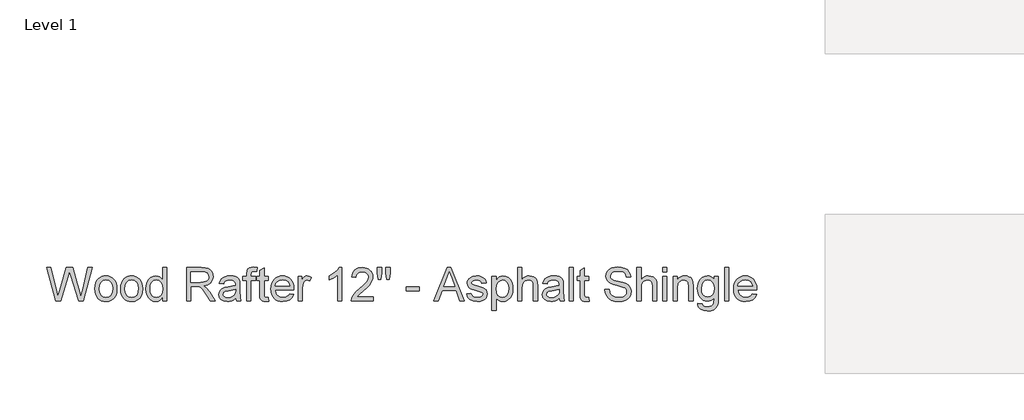
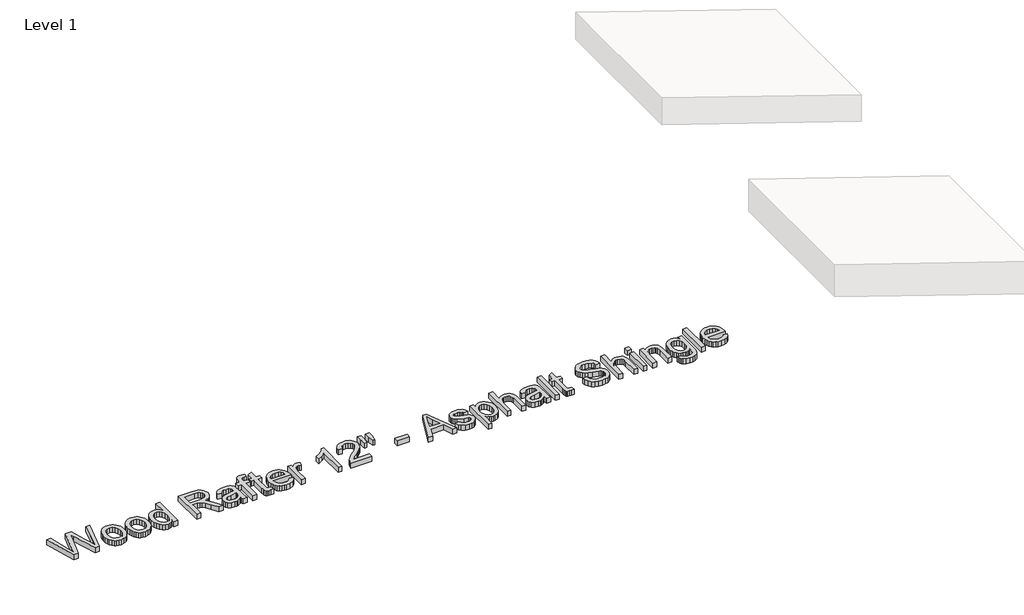
# One storey, part 5 of 42: 1 proxy.
"""IFC4 building model written with IfcOpenShell, lengths in millimetres."""

from ifc_helpers import new_model, si_unit, origin, origin_with_axes, place, context, project, spatial, polyline, outline, extrude, element, save

model = new_model("IFC4")

# Units and contexts
model_context = context("Model", 3, world=origin())
ifc_project = project(units=[si_unit("LENGTHUNIT", "METRE", prefix="MILLI")], contexts=[model_context])

# Site, building, storey
site = spatial("IfcSite", under=ifc_project)
building = spatial("IfcBuilding", under=site)
storey = spatial("IfcBuildingStorey", under=building, Name="Level 1", Elevation=0.0)

# Proxy
placement = place(None, origin())
element("IfcBuildingElementProxy", 1, Name="8\" Arial", ObjectType="8\" Arial", at=placement, inside=storey, context=model_context, shape_type="SweptSolid", body=[
    extrude(outline(polyline([(-8359.7335066, -14494.3519228), (-8442.7904998, -14189.7848287), (-8403.5298978, -14189.7848287), (-8355.3464318, -14389.954413), (-8340.4749916, -14451.7452468), (-8324.5625507, -14397.0927043), (-8264.1845037, -14189.7848287), (-8207.598674, -14189.7848287), (-8163.7279256, -14340.0607313), (-8144.9341431, -14395.8286318), (-8131.0851145, -14451.7452468), (-8116.6598175, -14391.7389858), (-8068.0302083, -14189.7848287), (-8028.7696063, -14189.7848287), (-8111.9009567, -14494.3519228), (-8152.5743455, -14494.3519228), (-8225.5931165, -14259.3831686), (-8235.780053, -14226.591643), (-8247.231062, -14266.0753166), (-8313.7807566, -14494.3519228), (-8359.7335066, -14494.3519228)])), origin_with_axes(), (0.0, 0.0, 1.0), 50.8),
    extrude(outline(polyline([(-8004.9753021, -14382.5186929), (-8002.9165371, -14353.5519159), (-7996.7402421, -14328.5911331), (-7986.4464171, -14307.6363445), (-7972.0350622, -14290.6875501), (-7957.5261134, -14279.8546354), (-7941.5114313, -14272.1168392), (-7923.9910159, -14267.4741615), (-7904.9648671, -14265.9266022), (-7883.9612816, -14267.8110925), (-7864.9699878, -14273.4645634), (-7847.9909858, -14282.887015), (-7833.0242754, -14296.0784471), (-7820.8087816, -14312.5927166), (-7812.0834288, -14331.9836804), (-7806.8482171, -14354.2513383), (-7805.1031466, -14379.3956905), (-7808.1889704, -14417.8569525), (-7817.4464419, -14447.1351003), (-7832.6060162, -14469.0611799), (-7853.3981484, -14485.4662373), (-7878.0940337, -14495.699647), (-7904.9648671, -14499.1107836), (-7926.2751761, -14497.2332643), (-7945.4430683, -14491.6007063), (-7962.4685436, -14482.2131098), (-7977.351602, -14469.0704745), (-7989.4369708, -14452.3958723), (-7998.0693771, -14432.4123746), (-8003.2488208, -14409.1199815), (-8004.9753021, -14382.5186929)]), holes=[polyline([(-7966.9044153, -14382.4443357), (-7962.4987512, -14416.8996036), (-7949.2817587, -14441.4467745), (-7929.3912076, -14456.1416163), (-7904.9648671, -14461.0398969), (-7880.6500625, -14456.1137323), (-7860.7966899, -14441.3352387), (-7847.5796975, -14416.462755), (-7843.1740333, -14381.2546205), (-7847.6075814, -14347.8031748), (-7860.9082257, -14323.5906114), (-7880.7894822, -14308.8957696), (-7904.9648671, -14303.997489), (-7929.3912076, -14308.8771803), (-7949.2817587, -14323.5162542), (-7962.4987512, -14348.0076571), (-7966.9044153, -14382.4443357)])]), origin_with_axes(), (0.0, 0.0, 1.0), 50.8),
    extrude(outline(polyline([(-7771.7911207, -14382.5186929), (-7769.7323557, -14353.5519159), (-7763.5560607, -14328.5911331), (-7753.2622357, -14307.6363445), (-7738.8508808, -14290.6875501), (-7724.341932, -14279.8546354), (-7708.3272499, -14272.1168392), (-7690.8068345, -14267.4741615), (-7671.7806857, -14265.9266022), (-7650.7771002, -14267.8110925), (-7631.7858064, -14273.4645634), (-7614.8068044, -14282.887015), (-7599.8400941, -14296.0784471), (-7587.6246002, -14312.5927166), (-7578.8992474, -14331.9836804), (-7573.6640357, -14354.2513383), (-7571.9189652, -14379.3956905), (-7575.004789, -14417.8569525), (-7584.2622605, -14447.1351003), (-7599.4218348, -14469.0611799), (-7620.213967, -14485.4662373), (-7644.9098523, -14495.699647), (-7671.7806857, -14499.1107836), (-7693.0909947, -14497.2332643), (-7712.2588869, -14491.6007063), (-7729.2843622, -14482.2131098), (-7744.1674206, -14469.0704745), (-7756.2527894, -14452.3958723), (-7764.8851957, -14432.4123746), (-7770.0646394, -14409.1199815), (-7771.7911207, -14382.5186929)]), holes=[polyline([(-7733.7202339, -14382.4443357), (-7729.3145698, -14416.8996036), (-7716.0975773, -14441.4467745), (-7696.2070262, -14456.1416163), (-7671.7806857, -14461.0398969), (-7647.4658811, -14456.1137323), (-7627.6125085, -14441.3352387), (-7614.3955161, -14416.462755), (-7609.9898519, -14381.2546205), (-7614.4234, -14347.8031748), (-7627.7240443, -14323.5906114), (-7647.6053009, -14308.8957696), (-7671.7806857, -14303.997489), (-7696.2070262, -14308.8771803), (-7716.0975773, -14323.5162542), (-7729.3145698, -14348.0076571), (-7733.7202339, -14382.4443357)])]), origin_with_axes(), (0.0, 0.0, 1.0), 50.8),
    extrude(outline(polyline([(-7391.0822531, -14494.3519228), (-7391.0822531, -14458.4373948), (-7402.4728468, -14476.2320024), (-7416.2707548, -14488.9424364), (-7432.4759773, -14496.5686968), (-7451.0885141, -14499.1107836), (-7475.7007475, -14495.4301022), (-7498.2309793, -14484.3880579), (-7517.3036013, -14466.7561067), (-7531.5430052, -14443.3057045), (-7540.4101014, -14414.9849057), (-7543.3658001, -14382.7417645), (-7540.6424676, -14350.8982933), (-7532.4724702, -14322.1406459), (-7518.8651025, -14298.1046808), (-7499.8296591, -14280.4262564), (-7476.8068108, -14269.5515158), (-7451.2372285, -14265.9266022), (-7432.6107497, -14268.5198096), (-7416.1406297, -14276.2994317), (-7402.1800653, -14288.2244678), (-7391.0822531, -14303.253917), (-7391.0822531, -14189.7848287), (-7353.0113663, -14189.7848287), (-7353.0113663, -14494.3519228), (-7391.0822531, -14494.3519228)]), holes=[polyline([(-7505.2949134, -14382.5930501), (-7501.000785, -14417.0297287), (-7488.1184, -14441.5211317), (-7469.3989747, -14456.1602056), (-7447.5937256, -14461.0398969), (-7425.7977712, -14456.3832772), (-7407.552373, -14442.4134181), (-7395.1997831, -14418.8700694), (-7391.0822531, -14385.4929809), (-7395.2741403, -14349.0021847), (-7407.8498018, -14323.7021472), (-7426.5599325, -14308.9236535), (-7449.1552268, -14303.997489), (-7471.1835475, -14308.7284659), (-7489.233758, -14322.9213966), (-7501.2796245, -14347.3012637), (-7505.2949134, -14382.5930501)])]), origin_with_axes(), (0.0, 0.0, 1.0), 50.8),
    extrude(outline(polyline([(-7172.1746542, -14494.3519228), (-7172.1746542, -14189.7848287), (-7040.934195, -14189.7848287), (-7005.6609979, -14191.8389464), (-6979.998469, -14198.0012994), (-6961.2418651, -14209.3779511), (-6946.6864431, -14227.0749649), (-6937.3453198, -14249.0196337), (-6934.231612, -14273.1392507), (-6939.3901428, -14303.1423812), (-6954.8657352, -14328.0148648), (-6966.5886126, -14338.1506807), (-6981.1231217, -14346.2509683), (-7018.6270348, -14356.3449583), (-6996.9890894, -14372.6291852), (-6966.1308511, -14411.81543), (-6915.344883, -14494.3519228), (-6959.5874174, -14494.3519228), (-6999.2198054, -14431.2226594), (-7027.8473277, -14389.4339126), (-7047.9609505, -14369.6920758), (-7066.0669288, -14362.4422487), (-7088.1510174, -14361.1038191), (-7134.1037675, -14361.1038191), (-7134.1037675, -14494.3519228), (-7172.1746542, -14494.3519228)]), holes=[polyline([(-7134.1037675, -14323.0329324), (-7048.8904155, -14323.0329324), (-7024.4176018, -14321.6852081), (-7005.4286317, -14317.6420353), (-6991.1334598, -14310.6338691), (-6980.742041, -14300.3911647), (-6974.4123843, -14288.0013962), (-6972.3024987, -14274.5520375), (-6976.3270822, -14255.9813266), (-6988.4008327, -14241.01694), (-7009.1743756, -14231.1460216), (-7039.2983366, -14227.8557155), (-7134.1037675, -14227.8557155), (-7134.1037675, -14323.0329324)])]), origin_with_axes(), (0.0, 0.0, 1.0), 50.8),
    extrude(outline(polyline([(-6729.6005957, -14465.7987577), (-6747.7902259, -14481.3951805), (-6766.5189458, -14491.6007063), (-6786.2143093, -14497.2332643), (-6807.3038704, -14499.1107836), (-6839.1194576, -14494.5935837), (-6862.5884491, -14481.0419838), (-6877.0602193, -14460.4636286), (-6881.8841427, -14434.8661622), (-6880.0623913, -14419.0838464), (-6874.597137, -14404.7514959), (-6866.1668894, -14392.4825578), (-6855.4501578, -14382.8904789), (-6828.7931014, -14370.3984692), (-6795.8528615, -14364.6729647), (-6756.9268669, -14358.6500315), (-6729.8236673, -14351.5860974), (-6729.6005957, -14343.1093765), (-6732.221687, -14326.1187562), (-6740.084961, -14315.0023547), (-6757.6704389, -14306.7487054), (-6782.1711366, -14303.997489), (-6804.8500828, -14305.828535), (-6820.6881665, -14311.3216732), (-6831.4885499, -14321.4807258), (-6839.0543951, -14337.3095149), (-6877.1252818, -14332.550654), (-6870.5167856, -14311.7306379), (-6860.6551619, -14295.3720537), (-6846.6202403, -14282.8614547), (-6827.4918504, -14273.5853939), (-6804.0972161, -14267.8413001), (-6777.2635613, -14265.9266022), (-6751.5266752, -14267.6182285), (-6731.1249183, -14272.6931075), (-6715.7422724, -14280.3240152), (-6705.0627194, -14289.6837278), (-6697.9801961, -14301.2555672), (-6693.3886389, -14315.5228551), (-6691.5297089, -14348.834881), (-6691.5297089, -14396.2004178), (-6689.5964217, -14462.3411479), (-6682.0119872, -14494.3519228), (-6720.082874, -14494.3519228), (-6726.1801644, -14481.116341), (-6729.6005957, -14465.7987577)]), holes=[polyline([(-6729.6005957, -14389.6569842), (-6791.0196434, -14401.3310647), (-6823.7739903, -14407.5027124), (-6838.6082519, -14417.5409344), (-6843.8132559, -14432.189303), (-6840.9783877, -14443.5101868), (-6832.4737828, -14452.7862476), (-6818.4853344, -14458.9764845), (-6799.1989355, -14461.0398969), (-6778.7507053, -14458.7627076), (-6760.6819056, -14451.9311398), (-6746.033537, -14441.8650337), (-6735.8466005, -14429.8842298), (-6731.3294006, -14417.5409344), (-6729.8236673, -14400.4387783), (-6729.6005957, -14389.6569842)])]), origin_with_axes(), (0.0, 0.0, 1.0), 50.8),
    extrude(outline(polyline([(-6629.6645179, -14494.3519228), (-6629.6645179, -14308.7563498), (-6662.9765438, -14308.7563498), (-6662.9765438, -14270.6854631), (-6629.6645179, -14270.6854631), (-6629.6645179, -14248.1552313), (-6625.6492291, -14216.4047066), (-6617.9904374, -14203.7453931), (-6606.1676425, -14193.7257603), (-6589.6231653, -14187.200916), (-6567.7993269, -14185.0259679), (-6533.0745142, -14189.1899711), (-6538.6513043, -14224.8814274), (-6560.5866785, -14223.0968546), (-6575.0584487, -14224.6769451), (-6584.5668757, -14229.4172167), (-6589.8369423, -14238.4702059), (-6591.5936312, -14252.9884493), (-6591.5936312, -14270.6854631), (-6548.7638836, -14270.6854631), (-6548.7638836, -14308.7563498), (-6591.5936312, -14308.7563498), (-6591.5936312, -14494.3519228), (-6629.6645179, -14494.3519228)])), origin_with_axes(), (0.0, 0.0, 1.0), 50.8),
    extrude(outline(polyline([(-6434.5512233, -14462.6013981), (-6429.7923624, -14495.4672808), (-6458.2711703, -14499.1107836), (-6476.5444524, -14497.5306931), (-6490.1704094, -14492.7904216), (-6499.7996669, -14485.4848266), (-6506.0828504, -14476.2087658), (-6509.5404602, -14460.2777355), (-6510.6929968, -14433.0072322), (-6510.6929968, -14308.7563498), (-6539.2461619, -14308.7563498), (-6539.2461619, -14270.6854631), (-6510.6929968, -14270.6854631), (-6510.6929968, -14216.3303494), (-6472.62211, -14193.9488319), (-6472.62211, -14270.6854631), (-6434.5512233, -14270.6854631), (-6434.5512233, -14308.7563498), (-6472.62211, -14308.7563498), (-6472.62211, -14431.8918742), (-6470.6144656, -14451.5221752), (-6464.1082106, -14458.4745734), (-6451.132879, -14461.0398969), (-6434.5512233, -14462.6013981)])), origin_with_axes(), (0.0, 0.0, 1.0), 50.8),
    extrude(outline(polyline([(-6239.8840718, -14427.7278709), (-6202.5567571, -14432.4867318), (-6216.0061158, -14460.612343), (-6237.4674628, -14481.6368415), (-6266.4574764, -14494.7422981), (-6302.4928348, -14499.1107836), (-6326.115188, -14497.2262933), (-6347.1629232, -14491.5728224), (-6365.6360402, -14482.1503709), (-6381.5345392, -14468.9589387), (-6394.3193304, -14452.3656647), (-6403.4513241, -14432.7376873), (-6408.9305203, -14410.0750068), (-6410.7569191, -14384.3776229), (-6408.911931, -14357.8088657), (-6403.3769669, -14334.3909948), (-6394.1520267, -14314.1240102), (-6381.2371104, -14297.0079121), (-6365.3804373, -14283.409839), (-6347.3302269, -14273.6969297), (-6327.086479, -14267.8691841), (-6304.6491937, -14265.9266022), (-6282.9345674, -14267.8645368), (-6263.2972954, -14273.6783404), (-6245.7373777, -14283.3680131), (-6230.2548144, -14296.9335549), (-6217.6164139, -14314.0124744), (-6208.588985, -14334.2422804), (-6203.1725277, -14357.6229727), (-6201.3670419, -14384.1545513), (-6201.5901135, -14394.415845), (-6372.6860323, -14394.415845), (-6366.0961254, -14422.9132422), (-6350.7878367, -14443.8633835), (-6328.6944534, -14456.7457685), (-6301.7492628, -14461.0398969), (-6281.4869256, -14459.0508417), (-6264.4219481, -14453.0836764), (-6250.5543301, -14442.7666148), (-6239.8840718, -14427.7278709)]), holes=[polyline([(-6372.6860323, -14356.3449583), (-6239.4379286, -14356.3449583), (-6244.5871648, -14336.2313355), (-6254.6811548, -14321.8432171), (-6276.8767792, -14308.458921), (-6304.7979081, -14303.997489), (-6330.4604369, -14307.55734), (-6351.6801231, -14318.2368929), (-6366.4307328, -14334.8836112), (-6372.6860323, -14356.3449583)])]), origin_with_axes(), (0.0, 0.0, 1.0), 50.8),
    extrude(outline(polyline([(-6163.2961551, -14494.3519228), (-6163.2961551, -14270.6854631), (-6129.9841292, -14270.6854631), (-6129.9841292, -14303.7744174), (-6117.6780125, -14284.5902596), (-6106.3385394, -14273.2879651), (-6094.9618877, -14267.7669429), (-6082.5442352, -14265.9266022), (-6063.583149, -14268.8637116), (-6044.324634, -14277.6750399), (-6057.0397153, -14311.8049951), (-6070.4240114, -14305.9493655), (-6083.8083076, -14303.997489), (-6095.1756646, -14305.8750083), (-6105.3347172, -14311.5075662), (-6113.5418932, -14320.4676089), (-6119.0536207, -14332.3275824), (-6123.6823565, -14353.5937418), (-6125.2252684, -14376.7931885), (-6125.2252684, -14494.3519228), (-6163.2961551, -14494.3519228)])), origin_with_axes(), (0.0, 0.0, 1.0), 50.8),
    extrude(outline(polyline([(-5768.310705, -14494.3519228), (-5806.3815918, -14494.3519228), (-5806.3815918, -14257.0037381), (-5842.4448341, -14282.694151), (-5882.5233653, -14301.9154874), (-5882.5233653, -14265.9266022), (-5852.6224759, -14249.6609646), (-5826.7182862, -14230.3095031), (-5806.2979399, -14209.7311478), (-5792.8485812, -14189.7848287), (-5768.310705, -14189.7848287), (-5768.310705, -14494.3519228)])), origin_with_axes(), (0.0, 0.0, 1.0), 50.8),
    extrude(outline(polyline([(-5482.7790543, -14456.281036), (-5482.7790543, -14494.3519228), (-5682.6512098, -14494.3519228), (-5678.5615638, -14468.1038309), (-5669.1739672, -14447.5905382), (-5655.4364743, -14427.6906923), (-5635.5645125, -14406.8613815), (-5607.7735087, -14383.5596937), (-5566.6911553, -14347.0688975), (-5542.0417433, -14320.1330015), (-5529.7170373, -14298.2719845), (-5525.6088019, -14277.0058251), (-5529.484671, -14257.9424978), (-5541.1122783, -14242.0951194), (-5558.9858904, -14231.4155664), (-5581.599774, -14227.8557155), (-5605.347605, -14231.3319146), (-5623.7974854, -14241.760512), (-5635.7039322, -14258.3235784), (-5639.8214622, -14280.2031848), (-5677.892349, -14275.4443239), (-5674.6183085, -14255.7907863), (-5668.6627614, -14238.6189203), (-5660.0257078, -14223.9287258), (-5648.7071477, -14211.7202029), (-5634.9673312, -14202.1234767), (-5619.0665085, -14195.2686723), (-5580.7818448, -14189.7848287), (-5560.3777642, -14191.3091513), (-5542.2183416, -14195.8821192), (-5526.303577, -14203.5037322), (-5512.6334704, -14214.1739905), (-5501.654165, -14227.1028488), (-5493.811804, -14241.5002618), (-5489.1063874, -14257.3662295), (-5487.5379152, -14274.7007519), (-5489.2295415, -14292.9089714), (-5494.3044204, -14310.8011728), (-5503.3109364, -14329.0000977), (-5516.7974736, -14348.1284876), (-5538.2959993, -14370.9654429), (-5571.3384803, -14400.2900639), (-5615.1348716, -14436.9109852), (-5632.3113849, -14456.281036), (-5482.7790543, -14456.281036)])), origin_with_axes(), (0.0, 0.0, 1.0), 50.8),
    extrude(outline(polyline([(-5435.4135175, -14299.2386281), (-5444.7081676, -14240.4220824), (-5444.7081676, -14189.7848287), (-5406.6372808, -14189.7848287), (-5406.6372808, -14240.4220824), (-5414.9652873, -14299.2386281), (-5435.4135175, -14299.2386281)])), origin_with_axes(), (0.0, 0.0, 1.0), 50.8),
    extrude(outline(polyline([(-5359.4948156, -14299.2386281), (-5368.566394, -14240.4220824), (-5368.566394, -14189.7848287), (-5330.4955073, -14189.7848287), (-5330.4955073, -14240.4220824), (-5339.4183714, -14299.2386281), (-5359.4948156, -14299.2386281)])), origin_with_axes(), (0.0, 0.0, 1.0), 50.8),
    extrude(outline(polyline([(-5182.9708211, -14403.9335667), (-5182.9708211, -14365.86268), (-5063.9993, -14365.86268), (-5063.9993, -14403.9335667), (-5182.9708211, -14403.9335667)])), origin_with_axes(), (0.0, 0.0, 1.0), 50.8),
    extrude(outline(polyline([(-4932.9075551, -14494.3519228), (-4811.333532, -14189.7848287), (-4778.9137925, -14189.7848287), (-4657.3397693, -14494.3519228), (-4697.5670149, -14494.3519228), (-4732.440542, -14399.1747059), (-4857.8811396, -14399.1747059), (-4892.6803096, -14494.3519228), (-4932.9075551, -14494.3519228)]), holes=[polyline([(-4843.9019859, -14361.1038191), (-4746.3453386, -14361.1038191), (-4773.7831456, -14286.226118), (-4795.1236622, -14227.8557155), (-4814.0847484, -14279.6826843), (-4843.9019859, -14361.1038191)])]), origin_with_axes(), (0.0, 0.0, 1.0), 50.8),
    extrude(outline(polyline([(-4635.7018239, -14427.7278709), (-4597.6309372, -14422.9690101), (-4591.6265932, -14439.2532371), (-4580.0082806, -14451.2247464), (-4562.7016422, -14458.5861092), (-4539.6323206, -14461.0398969), (-4516.8418386, -14458.7905915), (-4500.8178619, -14452.0426756), (-4491.3373188, -14442.2647037), (-4488.1771377, -14430.9252306), (-4491.3559081, -14421.2216159), (-4500.8922191, -14413.8230744), (-4540.0784638, -14402.9669231), (-4597.4078656, -14384.3404443), (-4611.9168144, -14374.9807317), (-4622.4290636, -14362.5909631), (-4628.8144882, -14347.9611839), (-4630.9429631, -14331.8814392), (-4629.2327475, -14317.1308296), (-4624.1021006, -14303.5141672), (-4616.0157551, -14291.5705418), (-4605.4384433, -14281.8390432), (-4581.2351744, -14270.5739273), (-4548.4808275, -14265.9266022), (-4523.7012904, -14267.7948269), (-4502.1562915, -14273.3995009), (-4484.8310637, -14282.1922399), (-4472.71084, -14293.6246595), (-4464.6802623, -14308.5425729), (-4459.6239727, -14327.7917932), (-4497.6948594, -14332.550654), (-4502.5001935, -14320.5698501), (-4512.0086206, -14311.5447448), (-4526.3130871, -14305.8843029), (-4545.5065395, -14303.997489), (-4567.3675565, -14305.8006511), (-4581.9415678, -14311.2101374), (-4590.1394492, -14319.0176435), (-4592.8720763, -14328.0148648), (-4588.3362871, -14339.0940877), (-4574.1340618, -14347.4964514), (-4541.3425362, -14355.6013863), (-4485.4630999, -14373.5214716), (-4470.7031956, -14382.091139), (-4459.5124369, -14393.8209874), (-4452.4577975, -14408.7481955), (-4450.106251, -14426.9099417), (-4452.8667621, -14445.6851349), (-4461.1482953, -14463.3449701), (-4474.6348326, -14478.5045444), (-4493.0103558, -14489.7789549), (-4515.2059802, -14496.7778264), (-4540.152821, -14499.1107836), (-4578.5397259, -14494.612173), (-4606.5538013, -14481.116341), (-4625.2546372, -14458.7720022), (-4635.7018239, -14427.7278709)])), origin_with_axes(), (0.0, 0.0, 1.0), 50.8),
    extrude(outline(polyline([(-4407.2765034, -14580.011418), (-4407.2765034, -14270.6854631), (-4369.2056166, -14270.6854631), (-4369.2056166, -14308.0127778), (-4356.7879641, -14289.600076), (-4342.8831676, -14276.4481461), (-4326.6732978, -14268.5569882), (-4307.3404256, -14265.9266022), (-4281.5942449, -14269.6072837), (-4259.0826024, -14280.649328), (-4240.7535524, -14298.3835203), (-4227.5551493, -14322.1406459), (-4219.5803395, -14350.1918999), (-4216.9220696, -14380.8084773), (-4219.9242416, -14413.3676366), (-4228.9307575, -14442.4877753), (-4243.6534832, -14466.6910441), (-4263.8042846, -14484.4995937), (-4287.2732761, -14495.4579861), (-4311.9505721, -14499.1107836), (-4329.4523982, -14496.6662906), (-4345.076705, -14489.3328117), (-4358.4517065, -14478.2628835), (-4369.2056166, -14464.6090425), (-4369.2056166, -14580.011418), (-4407.2765034, -14580.011418)]), holes=[polyline([(-4369.2056166, -14384.3032657), (-4365.0880866, -14418.4332209), (-4352.7354967, -14442.3018823), (-4334.5086879, -14456.3553932), (-4312.7685013, -14461.0398969), (-4290.675118, -14456.1880895), (-4271.9835767, -14441.6326675), (-4259.2406114, -14416.8903089), (-4254.9929564, -14381.4776921), (-4259.1383703, -14347.53363), (-4271.5746121, -14323.3303612), (-4289.773537, -14308.830707), (-4311.2070001, -14303.997489), (-4332.724115, -14309.1374305), (-4351.6201387, -14324.557255), (-4364.8092471, -14349.7736407), (-4369.2056166, -14384.3032657)])]), origin_with_axes(), (0.0, 0.0, 1.0), 50.8),
    extrude(outline(polyline([(-4174.092322, -14494.3519228), (-4174.092322, -14189.7848287), (-4136.0214352, -14189.7848287), (-4136.0214352, -14301.766773), (-4122.0376342, -14286.0866983), (-4106.3343229, -14274.8866449), (-4088.9115013, -14268.1666129), (-4069.7691694, -14265.9266022), (-4046.7742051, -14268.3710952), (-4027.013779, -14275.7045741), (-4011.4545348, -14287.3507707), (-4001.063116, -14302.7334166), (-3995.2074864, -14323.8694509), (-3993.2556099, -14352.7758126), (-3993.2556099, -14494.3519228), (-4031.3264966, -14494.3519228), (-4031.3264966, -14356.7167443), (-4034.3565526, -14332.8852614), (-4043.4467204, -14316.5638559), (-4058.0950889, -14307.1390807), (-4077.7997471, -14303.997489), (-4093.8887864, -14306.1166692), (-4108.9925928, -14312.4742099), (-4121.5031918, -14322.4566641), (-4129.812609, -14335.4505849), (-4134.4692287, -14352.7200447), (-4136.0214352, -14375.5291161), (-4136.0214352, -14494.3519228), (-4174.092322, -14494.3519228)])), origin_with_axes(), (0.0, 0.0, 1.0), 50.8),
    extrude(outline(polyline([(-3798.1423152, -14465.7987577), (-3816.3319455, -14481.3951805), (-3835.0606654, -14491.6007063), (-3854.7560289, -14497.2332643), (-3875.84559, -14499.1107836), (-3907.6611772, -14494.5935837), (-3931.1301687, -14481.0419838), (-3945.6019389, -14460.4636286), (-3950.4258623, -14434.8661622), (-3948.6041109, -14419.0838464), (-3943.1388566, -14404.7514959), (-3934.708609, -14392.4825578), (-3923.9918774, -14382.8904789), (-3897.334821, -14370.3984692), (-3864.3945811, -14364.6729647), (-3825.4685865, -14358.6500315), (-3798.3653869, -14351.5860974), (-3798.1423152, -14343.1093765), (-3800.7634066, -14326.1187562), (-3808.6266805, -14315.0023547), (-3826.2121585, -14306.7487054), (-3850.7128561, -14303.997489), (-3873.3918024, -14305.828535), (-3889.2298861, -14311.3216732), (-3900.0302695, -14321.4807258), (-3907.5961147, -14337.3095149), (-3945.6670014, -14332.550654), (-3939.0585052, -14311.7306379), (-3929.1968815, -14295.3720537), (-3915.1619599, -14282.8614547), (-3896.03357, -14273.5853939), (-3872.6389357, -14267.8413001), (-3845.8052809, -14265.9266022), (-3820.0683948, -14267.6182285), (-3799.6666379, -14272.6931075), (-3784.283992, -14280.3240152), (-3773.604439, -14289.6837278), (-3766.5219157, -14301.2555672), (-3761.9303585, -14315.5228551), (-3760.0714285, -14348.834881), (-3760.0714285, -14396.2004178), (-3758.1381413, -14462.3411479), (-3750.5537068, -14494.3519228), (-3788.6245936, -14494.3519228), (-3794.721884, -14481.116341), (-3798.1423152, -14465.7987577)]), holes=[polyline([(-3798.1423152, -14389.6569842), (-3859.561363, -14401.3310647), (-3892.3157099, -14407.5027124), (-3907.1499715, -14417.5409344), (-3912.3549755, -14432.189303), (-3909.5201072, -14443.5101868), (-3901.0155024, -14452.7862476), (-3887.027054, -14458.9764845), (-3867.7406551, -14461.0398969), (-3847.2924249, -14458.7627076), (-3829.2236251, -14451.9311398), (-3814.5752566, -14441.8650337), (-3804.3883201, -14429.8842298), (-3799.8711202, -14417.5409344), (-3798.3653869, -14400.4387783), (-3798.1423152, -14389.6569842)])]), origin_with_axes(), (0.0, 0.0, 1.0), 50.8),
    extrude(outline(polyline([(-3707.7239592, -14494.3519228), (-3707.7239592, -14189.7848287), (-3669.6530724, -14189.7848287), (-3669.6530724, -14494.3519228), (-3707.7239592, -14494.3519228)])), origin_with_axes(), (0.0, 0.0, 1.0), 50.8),
    extrude(outline(polyline([(-3531.6461079, -14462.6013981), (-3526.8872471, -14495.4672808), (-3555.366055, -14499.1107836), (-3573.639337, -14497.5306931), (-3587.2652941, -14492.7904216), (-3596.8945516, -14485.4848266), (-3603.177735, -14476.2087658), (-3606.6353448, -14460.2777355), (-3607.7878815, -14433.0072322), (-3607.7878815, -14308.7563498), (-3636.3410465, -14308.7563498), (-3636.3410465, -14270.6854631), (-3607.7878815, -14270.6854631), (-3607.7878815, -14216.3303494), (-3569.7169947, -14193.9488319), (-3569.7169947, -14270.6854631), (-3531.6461079, -14270.6854631), (-3531.6461079, -14308.7563498), (-3569.7169947, -14308.7563498), (-3569.7169947, -14431.8918742), (-3567.7093503, -14451.5221752), (-3561.2030952, -14458.4745734), (-3548.2277637, -14461.0398969), (-3531.6461079, -14462.6013981)])), origin_with_axes(), (0.0, 0.0, 1.0), 50.8),
    extrude(outline(polyline([(-3384.1214218, -14389.6569842), (-3346.050535, -14389.6569842), (-3341.6820495, -14410.7837238), (-3333.7815969, -14427.7650495), (-3321.4568909, -14441.2422922), (-3303.815645, -14451.8567826), (-3282.2520568, -14458.7441183), (-3258.1603238, -14461.0398969), (-3236.9499323, -14459.3017973), (-3218.3792214, -14454.0874986), (-3203.3311829, -14445.8338493), (-3192.6888085, -14434.977698), (-3186.3591518, -14422.5135722), (-3184.2492663, -14409.4359996), (-3185.8293568, -14396.6930343), (-3190.5696283, -14385.6788739), (-3200.1988858, -14376.2819827), (-3216.4459342, -14368.3908248), (-3271.8792273, -14353.853992), (-3308.2677824, -14344.2340292), (-3331.5508809, -14335.0787989), (-3350.5026724, -14322.270771), (-3363.9334418, -14306.7487054), (-3371.9361355, -14288.8472093), (-3374.6037001, -14268.9008902), (-3371.3040993, -14246.6030247), (-3361.4052969, -14225.8108924), (-3345.1675432, -14208.1882359), (-3322.8510884, -14195.3987974), (-3296.0639068, -14187.6191752), (-3266.413973, -14185.0259679), (-3234.2916623, -14187.7400057), (-3206.1846405, -14195.8821192), (-3183.0967297, -14209.2850046), (-3166.0317521, -14227.7813583), (-3155.2313687, -14250.2186436), (-3150.9372404, -14275.4443239), (-3189.0081271, -14275.4443239), (-3195.997704, -14252.7281991), (-3210.5717153, -14236.3324363), (-3233.343608, -14226.40575), (-3264.926829, -14223.0968546), (-3297.253622, -14226.3685714), (-3319.4306571, -14236.1837219), (-3332.2572743, -14250.6276082), (-3336.5328133, -14267.7855322), (-3333.5027574, -14282.4153115), (-3324.4125896, -14294.1823385), (-3302.9233586, -14304.7038824), (-3262.2499698, -14315.4484979), (-3220.27533, -14325.6540237), (-3194.882346, -14334.5582985), (-3173.179338, -14348.3701485), (-3158.038353, -14365.4165368), (-3149.1433729, -14385.5115702), (-3146.1783795, -14408.469356), (-3149.5895161, -14431.9383474), (-3159.8229258, -14454.0131414), (-3176.4603495, -14473.0114062), (-3199.0835278, -14487.2508101), (-3226.2889686, -14496.1457902), (-3256.6731798, -14499.1107836), (-3293.9726106, -14495.913424), (-3324.6728398, -14486.3213451), (-3349.1270642, -14470.2973683), (-3367.6884804, -14447.8043151), (-3379.6042218, -14420.4036867), (-3384.1214218, -14389.6569842)])), origin_with_axes(), (0.0, 0.0, 1.0), 50.8),
    extrude(outline(polyline([(-3093.8309102, -14494.3519228), (-3093.8309102, -14189.7848287), (-3055.7600235, -14189.7848287), (-3055.7600235, -14301.766773), (-3041.7762224, -14286.0866983), (-3026.0729111, -14274.8866449), (-3008.6500895, -14268.1666129), (-2989.5077576, -14265.9266022), (-2966.5127933, -14268.3710952), (-2946.7523672, -14275.7045741), (-2931.193123, -14287.3507707), (-2920.8017042, -14302.7334166), (-2914.9460746, -14323.8694509), (-2912.9941981, -14352.7758126), (-2912.9941981, -14494.3519228), (-2951.0650849, -14494.3519228), (-2951.0650849, -14356.7167443), (-2954.0951408, -14332.8852614), (-2963.1853086, -14316.5638559), (-2977.8336771, -14307.1390807), (-2997.5383353, -14303.997489), (-3013.6273746, -14306.1166692), (-3028.731181, -14312.4742099), (-3041.24178, -14322.4566641), (-3049.5511972, -14335.4505849), (-3054.2078169, -14352.7200447), (-3055.7600235, -14375.5291161), (-3055.7600235, -14494.3519228), (-3093.8309102, -14494.3519228)])), origin_with_axes(), (0.0, 0.0, 1.0), 50.8),
    extrude(outline(polyline([(-2860.6467288, -14227.8557155), (-2860.6467288, -14189.7848287), (-2822.5758421, -14189.7848287), (-2822.5758421, -14227.8557155), (-2860.6467288, -14227.8557155)])), origin_with_axes(), (0.0, 0.0, 1.0), 50.8),
    extrude(outline(polyline([(-2860.6467288, -14494.3519228), (-2860.6467288, -14270.6854631), (-2822.5758421, -14270.6854631), (-2822.5758421, -14494.3519228), (-2860.6467288, -14494.3519228)])), origin_with_axes(), (0.0, 0.0, 1.0), 50.8),
    extrude(outline(polyline([(-2765.4695119, -14494.3519228), (-2765.4695119, -14270.6854631), (-2727.3986252, -14270.6854631), (-2727.3986252, -14301.9154874), (-2714.1723381, -14286.1703501), (-2698.2877811, -14274.9238235), (-2679.7449542, -14268.1759075), (-2658.5438573, -14265.9266022), (-2639.7779588, -14267.739059), (-2622.5921508, -14273.1764293), (-2608.2598003, -14281.5602037), (-2598.0542745, -14292.2118727), (-2586.6404442, -14320.2073587), (-2584.6327998, -14357.0141731), (-2584.6327998, -14494.3519228), (-2622.7036866, -14494.3519228), (-2622.7036866, -14362.1448199), (-2627.0907614, -14328.461008), (-2633.1601679, -14318.4320806), (-2642.5942378, -14310.6524584), (-2654.6865775, -14305.6612313), (-2668.7307938, -14303.997489), (-2691.0286594, -14307.7339383), (-2710.0362188, -14318.9432863), (-2717.6322716, -14328.0938693), (-2723.0580236, -14340.599821), (-2727.3986252, -14375.6778305), (-2727.3986252, -14494.3519228), (-2765.4695119, -14494.3519228)])), origin_with_axes(), (0.0, 0.0, 1.0), 50.8),
    extrude(outline(polyline([(-2541.8030522, -14513.3873661), (-2503.7321655, -14518.146227), (-2499.5309836, -14530.0433791), (-2491.3888701, -14538.2226712), (-2475.3834827, -14544.5802118), (-2454.4333414, -14546.6993921), (-2432.0890026, -14544.3013723), (-2415.4701682, -14537.1073132), (-2403.9448021, -14525.5819471), (-2396.8808681, -14510.1900065), (-2394.278366, -14465.7987577), (-2406.9469741, -14478.2907674), (-2421.0841369, -14487.2136315), (-2436.6898544, -14492.56735), (-2453.7641266, -14494.3519228), (-2474.637587, -14492.2745685), (-2493.0154339, -14486.0425056), (-2508.8976672, -14475.6557341), (-2522.284287, -14461.1142541), (-2532.9057484, -14443.6681958), (-2540.4925066, -14424.5676899), (-2545.0445614, -14403.8127363), (-2546.5619131, -14381.4033349), (-2543.8385806, -14350.6659271), (-2535.6685832, -14322.4008962), (-2522.3400549, -14298.4485829), (-2504.1411301, -14280.649328), (-2481.6945501, -14269.6072837), (-2455.6230566, -14265.9266022), (-2437.8191544, -14268.0086038), (-2421.6604052, -14274.2546087), (-2407.1468091, -14284.6646168), (-2394.278366, -14299.2386281), (-2394.278366, -14270.6854631), (-2356.2074793, -14270.6854631), (-2356.2074793, -14463.7911133), (-2358.8099813, -14508.3775498), (-2366.6174874, -14537.7393494), (-2380.066846, -14557.2116413), (-2399.5949059, -14572.1295547), (-2424.774113, -14581.6100978), (-2455.1769134, -14584.7702788), (-2490.5988249, -14580.3181414), (-2518.4920698, -14566.9617293), (-2528.9973481, -14556.9351255), (-2536.3842712, -14544.6638637), (-2540.6528393, -14530.1479439), (-2541.8030522, -14513.3873661)]), holes=[polyline([(-2508.4910263, -14378.8008329), (-2504.4292642, -14413.7208333), (-2492.243978, -14437.7289144), (-2473.9242226, -14451.6430056), (-2451.4590534, -14456.281036), (-2429.1611878, -14451.6708896), (-2410.748486, -14437.8404502), (-2398.395896, -14414.1390925), (-2394.278366, -14379.9161909), (-2398.5167265, -14346.9108884), (-2411.2318078, -14323.1444682), (-2429.9140545, -14308.7842338), (-2452.053911, -14303.997489), (-2473.7940975, -14308.7098766), (-2492.0209063, -14322.8470394), (-2504.3734963, -14346.2602629), (-2508.4910263, -14378.8008329)])]), origin_with_axes(), (0.0, 0.0, 1.0), 50.8),
    extrude(outline(polyline([(-2299.1011491, -14494.3519228), (-2299.1011491, -14189.7848287), (-2261.0302624, -14189.7848287), (-2261.0302624, -14494.3519228), (-2299.1011491, -14494.3519228)])), origin_with_axes(), (0.0, 0.0, 1.0), 50.8),
    extrude(outline(polyline([(-2047.3276676, -14427.7278709), (-2010.0003528, -14432.4867318), (-2023.4497115, -14460.612343), (-2044.9110585, -14481.6368415), (-2073.9010722, -14494.7422981), (-2109.9364306, -14499.1107836), (-2133.5587837, -14497.2262933), (-2154.6065189, -14491.5728224), (-2173.0796359, -14482.1503709), (-2188.9781349, -14468.9589387), (-2201.7629261, -14452.3656647), (-2210.8949198, -14432.7376873), (-2216.374116, -14410.0750068), (-2218.2005148, -14384.3776229), (-2216.3555267, -14357.8088657), (-2210.8205626, -14334.3909948), (-2201.5956224, -14314.1240102), (-2188.6807061, -14297.0079121), (-2172.824033, -14283.409839), (-2154.7738226, -14273.6969297), (-2134.5300747, -14267.8691841), (-2112.0927894, -14265.9266022), (-2090.3781631, -14267.8645368), (-2070.7408911, -14273.6783404), (-2053.1809735, -14283.3680131), (-2037.6984101, -14296.9335549), (-2025.0600096, -14314.0124744), (-2016.0325807, -14334.2422804), (-2010.6161234, -14357.6229727), (-2008.8106376, -14384.1545513), (-2009.0337092, -14394.415845), (-2180.129628, -14394.415845), (-2173.5397211, -14422.9132422), (-2158.2314324, -14443.8633835), (-2136.1380491, -14456.7457685), (-2109.1928585, -14461.0398969), (-2088.9305214, -14459.0508417), (-2071.8655438, -14453.0836764), (-2057.9979259, -14442.7666148), (-2047.3276676, -14427.7278709)]), holes=[polyline([(-2180.129628, -14356.3449583), (-2046.8815244, -14356.3449583), (-2052.0307605, -14336.2313355), (-2062.1247505, -14321.8432171), (-2084.3203749, -14308.458921), (-2112.2415038, -14303.997489), (-2137.9040327, -14307.55734), (-2159.1237188, -14318.2368929), (-2173.8743285, -14334.8836112), (-2180.129628, -14356.3449583)])]), origin_with_axes(), (0.0, 0.0, 1.0), 50.8),
])

save(model, "model.ifc")

# Revit data of these elements
# Element 1 (IfcBuildingElementProxy, "8\" Arial")
#   Phase Created = New Construction
